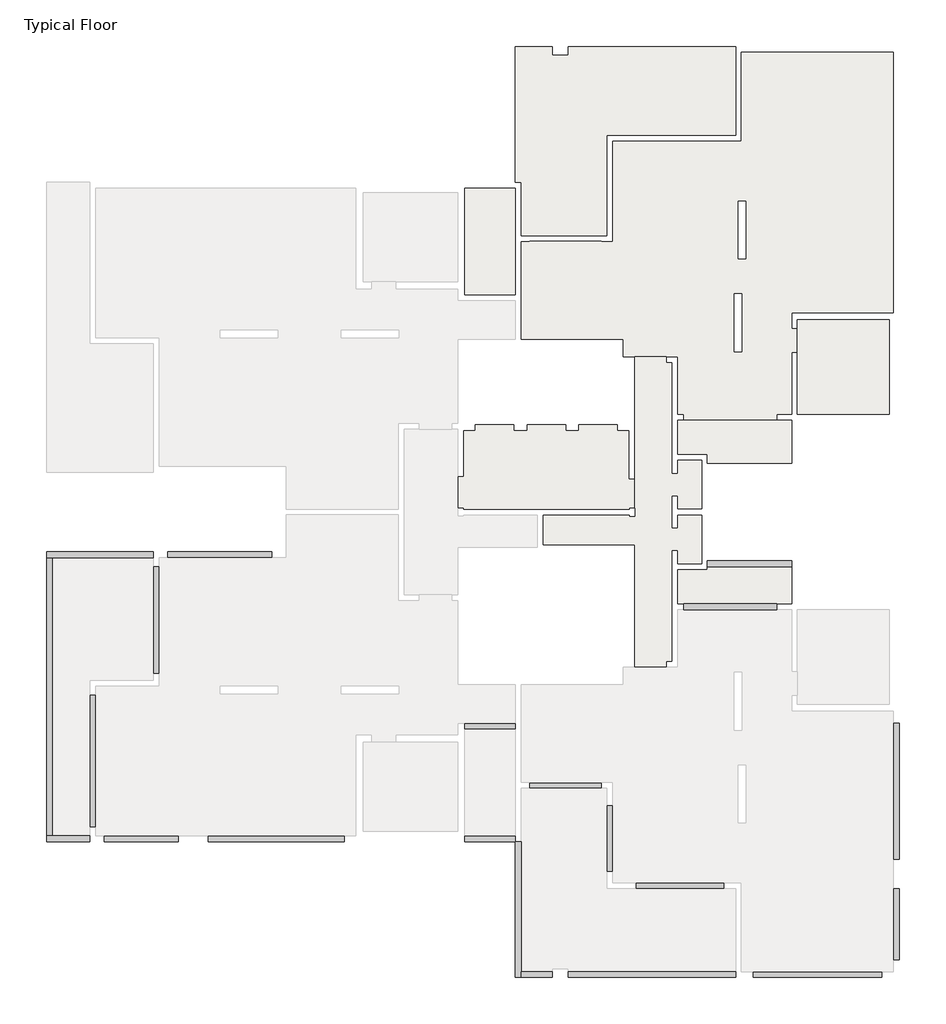
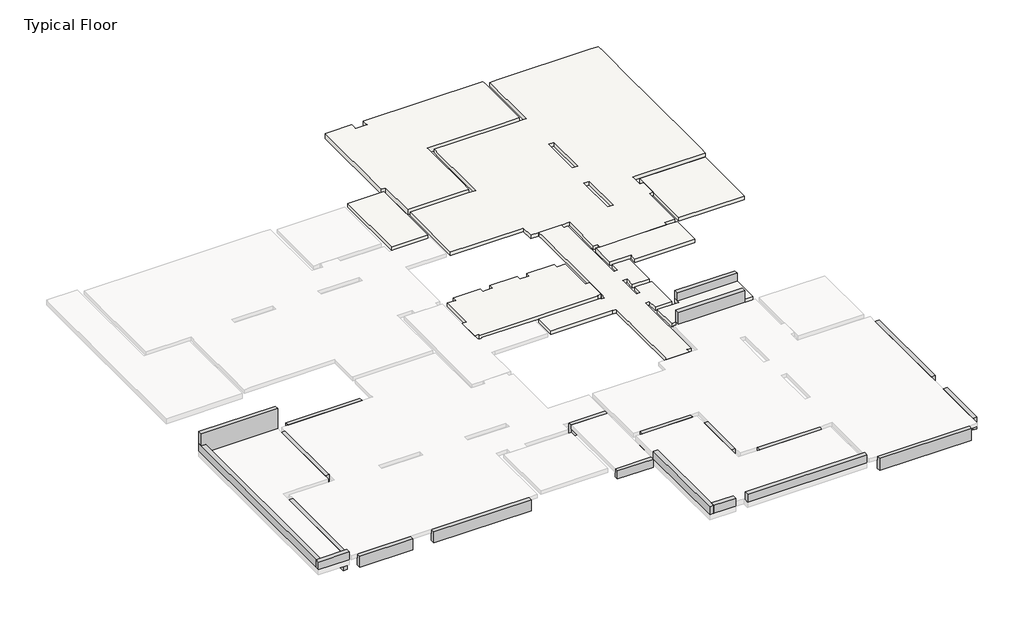
# One storey, part 2 of 2: 21 beams, 8 slabs.
"""IFC4 building model written with IfcOpenShell, lengths in millimetres."""

from ifc_helpers import new_model, si_unit, frame, origin, place, context, project, spatial, polyline, outline, extrude, faceted_brep, element, save

model = new_model("IFC4")

# Units and contexts
model_context = context("Model", 3, world=origin())
ifc_project = project(units=[si_unit("LENGTHUNIT", "METRE", prefix="MILLI")], contexts=[model_context])

# Site, building, storey
site = spatial("IfcSite", under=ifc_project)
building = spatial("IfcBuilding", under=site)
storey = spatial("IfcBuildingStorey", under=building, Name="Typical Floor", Elevation=3000.0)

# Beams
placement = place(None, origin())
element("IfcBeam", 1, ObjectType="Concrete Rectengular Beam : 20/40", at=placement, inside=storey, context=model_context, shape_type="Brep", body=[
    faceted_brep([(2246.4257984, -7661.3958819, 3000.0), (2246.4257984, -7661.3958819, 3400.0), (2446.4257984, -7661.3958819, 3400.0), (2446.4257984, -7661.3958819, 3000.0), (2246.4257984, -12260.9784014, 3400.0), (2446.4257984, -12260.9784014, 3400.0), (2446.4257984, -12060.9784014, 3400.0), (2446.4257984, -12260.9784014, 3000.0), (2446.4257984, -12060.9784014, 3000.0), (2246.4257984, -12260.9784014, 3000.0)], [[[0, 1, 2, 3]], [[2, 1, 4, 5, 6]], [[3, 2, 6, 5, 7, 8]], [[0, 3, 8, 7, 9]], [[1, 0, 9, 4]], [[5, 4, 9, 7]]]),
])
element("IfcBeam", 2, ObjectType="Concrete Rectengular Beam : 20/40", at=placement, inside=storey, context=model_context, shape_type="SweptSolid", body=[
    extrude(outline(polyline([(3495.6958179, -12060.9784014), (3495.6958179, -12260.9784014), (2446.4257984, -12260.9784014), (2446.4257984, -12060.9784014), (3495.6958179, -12060.9784014)])), frame((0.0, 0.0, 3000.0), z_axis=(0.0, 0.0, 1.0), x_axis=(1.0, 0.0, 0.0)), (0.0, 0.0, 1.0), 400.0),
])
element("IfcBeam", 3, ObjectType="Concrete Rectengular Beam : 20/40", at=placement, inside=storey, context=model_context, shape_type="SweptSolid", body=[
    extrude(outline(polyline([(9702.4292163, -12261.3104327), (4045.6958179, -12261.3104327), (4045.6958179, -12061.3104327), (9702.4292163, -12061.3104327), (9702.4292163, -12261.3104327)])), frame((0.0, 0.0, 3000.0), z_axis=(0.0, 0.0, 1.0), x_axis=(1.0, 0.0, 0.0)), (0.0, 0.0, 1.0), 400.0),
])
element("IfcBeam", 4, ObjectType="Concrete Rectengular Beam : 20/40", at=placement, inside=storey, context=model_context, shape_type="Brep", body=[
    faceted_brep([(2246.4257984, -7661.3958819, 3000.0), (2246.4257984, -7461.3958819, 3000.0), (542.9516773, -7461.3958819, 3000.0), (542.9516773, -7661.3958819, 3000.0), (542.9516773, -7661.3958819, 2600.0), (2246.4257984, -7661.3958819, 2600.0), (2246.4257984, -7461.3958819, 2600.0), (542.9516773, -7461.3958819, 2600.0), (2246.4257984, -7461.3958819, 2820.0), (542.9516773, -7461.3958819, 2820.0)], [[[0, 1, 2, 3]], [[3, 4, 5, 0]], [[6, 5, 4, 7]], [[1, 8, 6, 7, 9, 2]], [[1, 0, 5, 6, 8]], [[3, 2, 9, 7, 4]]]),
])
element("IfcBeam", 5, ObjectType="Concrete Rectengular Beam : 20/40", at=placement, inside=storey, context=model_context, shape_type="Brep", body=[
    faceted_brep([(-12154.2455884, -7461.3958819, 3000.0), (-12154.2455884, -7461.3958819, 3400.0), (-12154.2455884, -7661.3958819, 3400.0), (-12154.2455884, -7661.3958819, 3000.0), (-13414.2455884, -7461.3958819, 3400.0), (-13614.2455884, -7461.3958819, 3400.0), (-13614.2455884, -7661.3958819, 3400.0), (-13614.2455884, -7661.3958819, 3000.0), (-13614.2455884, -7461.3958819, 3000.0), (-13414.2455884, -7461.3958819, 3000.0)], [[[0, 1, 2, 3]], [[2, 1, 4, 5, 6]], [[3, 2, 6, 7]], [[0, 3, 7, 8, 9]], [[1, 0, 9, 8, 5, 4]], [[6, 5, 8, 7]]]),
])
element("IfcBeam", 6, ObjectType="Concrete Rectengular Beam : 20/40", at=placement, inside=storey, context=model_context, shape_type="Brep", body=[
    faceted_brep([(-13414.2455884, 2140.1763837, 3400.0), (-13614.2455884, 2140.1763837, 3400.0), (-13614.2455884, 1940.1763837, 3400.0), (-13614.2455884, -7461.3958819, 3400.0), (-13414.2455884, -7461.3958819, 3400.0), (-13414.2455884, 1940.1763837, 3400.0), (-13614.2455884, 2140.1763837, 3000.0), (-13614.2455884, -7461.3958819, 3000.0), (-13414.2455884, 2140.1763837, 3000.0), (-13414.2455884, 1940.1763837, 3000.0), (-13414.2455884, -7461.3958819, 3000.0)], [[[0, 1, 2, 3, 4, 5]], [[1, 6, 7, 3, 2]], [[6, 8, 9, 10, 7]], [[8, 0, 5, 4, 10, 9]], [[4, 3, 7, 10]], [[1, 0, 8, 6]]]),
])
element("IfcBeam", 7, ObjectType="Concrete Rectengular Beam : 20/40", at=placement, inside=storey, context=model_context, shape_type="SweptSolid", body=[
    extrude(outline(polyline([(8750.5859546, 1845.1910322), (11596.5527515, 1845.1910322), (11596.5527515, 1645.1910322), (8750.5859546, 1645.1910322), (8750.5859546, 1845.1910322)])), frame((0.0, 0.0, 3000.0), z_axis=(0.0, 0.0, 1.0), x_axis=(1.0, 0.0, 0.0)), (0.0, 0.0, 1.0), 400.0),
])
element("IfcBeam", 8, ObjectType="Concrete Rectengular Beam : 20/55", at=placement, inside=storey, context=model_context, shape_type="SweptSolid", body=[
    extrude(outline(polyline([(-7661.3958819, 2450.0), (-7661.3958819, 3000.0), (-7466.3958819, 3000.0), (-7466.3958819, 2820.0), (-7461.3958819, 2820.0), (-7461.3958819, 2450.0), (-7661.3958819, 2450.0)])), frame((-11654.2455884, 0.0, 0.0), z_axis=(1.0, 0.0, 0.0), x_axis=(0.0, 1.0, 0.0)), (0.0, 0.0, 1.0), 2499.5068359),
])
element("IfcBeam", 9, ObjectType="Concrete Rectengular Beam : 20/55", at=placement, inside=storey, context=model_context, shape_type="SweptSolid", body=[
    extrude(outline(polyline([(-7461.3958819, 2450.0), (-7661.3958819, 2450.0), (-7661.3958819, 3000.0), (-7466.3958819, 3000.0), (-7466.3958819, 2820.0), (-7461.3958819, 2820.0), (-7461.3958819, 2450.0)])), frame((-8149.7387524, 0.0, 0.0), z_axis=(1.0, 0.0, 0.0), x_axis=(0.0, 1.0, 0.0)), (0.0, 0.0, 1.0), 4602.6904297),
])
element("IfcBeam", 10, ObjectType="Concrete Rectengular Beam : 20/60", at=placement, inside=storey, context=model_context, shape_type="SweptSolid", body=[
    extrude(outline(polyline([(15247.1826343, -11661.3104327), (15047.1826343, -11661.3104327), (15047.1826343, -9252.3065264), (15247.1826343, -9252.3065264), (15247.1826343, -11661.3104327)])), frame((0.0, 0.0, 2400.0), z_axis=(0.0, 0.0, 1.0), x_axis=(1.0, 0.0, 0.0)), (0.0, 0.0, 1.0), 600.0),
])
element("IfcBeam", 11, ObjectType="Concrete Rectengular Beam : 20/60", at=placement, inside=storey, context=model_context, shape_type="SweptSolid", body=[
    extrude(outline(polyline([(15247.1826343, -8260.429085), (15047.1826343, -8260.429085), (15047.1826343, -3654.8187334), (15247.1826343, -3654.8187334), (15247.1826343, -8260.429085)])), frame((0.0, 0.0, 2400.0), z_axis=(0.0, 0.0, 1.0), x_axis=(1.0, 0.0, 0.0)), (0.0, 0.0, 1.0), 600.0),
])
element("IfcBeam", 12, ObjectType="Concrete Rectengular Beam : 20/60", at=placement, inside=storey, context=model_context, shape_type="Brep", body=[
    faceted_brep([(2246.4257984, -3861.3299639, 3000.0), (2246.4257984, -3661.3299639, 3000.0), (542.9516773, -3661.3299639, 3000.0), (542.9516773, -3861.3299639, 3000.0), (2246.4257984, -3861.3299639, 2400.0), (2246.4257984, -3861.3299639, 2820.0), (542.9516773, -3861.3299639, 2820.0), (542.9516773, -3861.3299639, 2400.0), (2246.4257984, -3661.3299639, 2400.0), (542.9516773, -3661.3299639, 2400.0), (2246.4257984, -3661.3299639, 2820.0)], [[[0, 1, 2, 3]], [[4, 5, 0, 3, 6, 7]], [[8, 4, 7, 9]], [[1, 10, 8, 9, 2]], [[1, 0, 5, 4, 8, 10]], [[3, 2, 9, 7, 6]]]),
])
element("IfcBeam", 13, ObjectType="Concrete Rectengular Beam : 20/60", at=placement, inside=storey, context=model_context, shape_type="SweptSolid", body=[
    extrude(outline(polyline([(11103.869646, 188.6553877), (7955.5859546, 188.6553877), (7955.5859546, 388.6553877), (11103.869646, 388.6553877), (11103.869646, 188.6553877)])), frame((0.0, 0.0, 3000.0), z_axis=(0.0, 0.0, 1.0), x_axis=(1.0, 0.0, 0.0)), (0.0, 0.0, 1.0), 600.0),
])
element("IfcBeam", 14, ObjectType="Concrete Rectengular Beam : 20/60", at=placement, inside=storey, context=model_context, shape_type="SweptSolid", body=[
    extrude(outline(polyline([(-12061.3104327, 2400.0), (-12261.3104327, 2400.0), (-12261.3104327, 3000.0), (-12066.3104327, 3000.0), (-12066.3104327, 2820.0), (-12061.3104327, 2820.0), (-12061.3104327, 2400.0)])), frame((10302.4292163, 0.0, 0.0), z_axis=(1.0, 0.0, 0.0), x_axis=(0.0, 1.0, 0.0)), (0.0, 0.0, 1.0), 4350.0610352),
])
element("IfcBeam", 15, ObjectType="Concrete Rectengular Beam : 20/85", at=placement, inside=storey, context=model_context, shape_type="Brep", body=[
    faceted_brep([(-12154.2455884, -7161.3958819, 3000.0), (-11954.2455884, -7161.3958819, 3000.0), (-11954.2455884, -2706.3494952, 3000.0), (-12154.2455884, -2706.3494952, 3000.0), (-11954.2455884, -7161.3958819, 2150.0), (-11954.2455884, -2706.3494952, 2150.0), (-12154.2455884, -7161.3958819, 2150.0), (-12154.2455884, -2706.3494952, 2150.0), (-12154.2455884, -2706.3494952, 2750.0), (-12154.2455884, -7161.3958819, 2750.0)], [[[0, 1, 2, 3]], [[1, 4, 5, 2]], [[4, 6, 7, 5]], [[0, 3, 8, 7, 6, 9]], [[1, 0, 9, 6, 4]], [[3, 2, 5, 7, 8]]]),
])
element("IfcBeam", 16, ObjectType="Concrete Rectengular Beam : 20/85", at=placement, inside=storey, context=model_context, shape_type="SweptSolid", body=[
    extrude(outline(polyline([(-5660.2777178, 2150.0), (-5860.2777178, 2150.0), (-5860.2777178, 3000.0), (-5665.2777178, 3000.0), (-5665.2777178, 2820.0), (-5660.2777178, 2820.0), (-5660.2777178, 2150.0)])), frame((2745.6201343, 0.0, 0.0), z_axis=(1.0, 0.0, 0.0), x_axis=(0.0, 1.0, 0.0)), (0.0, 0.0, 1.0), 2406.9848633),
])
element("IfcBeam", 17, ObjectType="Concrete Rectengular Beam : 20/85", at=placement, inside=storey, context=model_context, shape_type="Brep", body=[
    faceted_brep([(5545.4492359, -6456.8182452, 3000.0), (5345.4492359, -6456.8182452, 3000.0), (5345.4492359, -8661.9549639, 3000.0), (5545.4492359, -8661.9549639, 3000.0), (5545.4492359, -6456.8182452, 2150.0), (5545.4492359, -6456.8182452, 2820.0), (5545.4492359, -8661.9549639, 2820.0), (5545.4492359, -8661.9549639, 2150.0), (5345.4492359, -6456.8182452, 2150.0), (5345.4492359, -8661.9549639, 2150.0), (5345.4492359, -6456.8182452, 2750.0), (5345.4492359, -8661.9549639, 2750.0)], [[[0, 1, 2, 3]], [[4, 5, 0, 3, 6, 7]], [[8, 4, 7, 9]], [[2, 1, 10, 8, 9, 11]], [[1, 0, 5, 4, 8, 10]], [[3, 2, 11, 9, 7, 6]]]),
])
element("IfcBeam", 18, ObjectType="Concrete Rectengular Beam : 20/85", at=placement, inside=storey, context=model_context, shape_type="Brep", body=[
    faceted_brep([(6350.1123218, -9061.9549639, 3000.0), (6350.1123218, -9261.9549639, 3000.0), (9302.4292163, -9261.9549639, 3000.0), (9302.4292163, -9061.9549639, 3000.0), (9302.4292163, -9061.9549639, 2820.0), (9302.4292163, -9061.9549639, 2150.0), (6350.1123218, -9061.9549639, 2150.0), (6350.1123218, -9061.9549639, 2820.0), (6350.1123218, -9261.9549639, 2150.0), (9302.4292163, -9261.9549639, 2150.0), (6350.1123218, -9261.9549639, 2750.0), (9302.4292163, -9261.9549639, 2750.0)], [[[0, 1, 2, 3]], [[0, 3, 4, 5, 6, 7]], [[8, 6, 5, 9]], [[2, 1, 10, 8, 9, 11]], [[1, 0, 7, 6, 8, 10]], [[3, 2, 11, 9, 5, 4]]]),
])
element("IfcBeam", 19, ObjectType="Concrete Rectengular Beam : 20/85", at=placement, inside=storey, context=model_context, shape_type="Brep", body=[
    faceted_brep([(-9805.5395337, 1640.1763837, 3000.0), (-10005.5395337, 1640.1763837, 3000.0), (-10005.5395337, -1959.7284014, 3000.0), (-9805.5395337, -1959.7284014, 3000.0), (-10005.5395337, 1640.1763837, 2150.0), (-10005.5395337, -1959.7284014, 2150.0), (-9805.5395337, 1640.1763837, 2150.0), (-9805.5395337, -1959.7284014, 2150.0), (-9805.5395337, -1959.7284014, 2820.0), (-9805.5395337, 1640.1763837, 2820.0)], [[[0, 1, 2, 3]], [[1, 4, 5, 2]], [[4, 6, 7, 5]], [[0, 3, 8, 7, 6, 9]], [[1, 0, 9, 6, 4]], [[3, 2, 5, 7, 8]]]),
])
element("IfcBeam", 20, ObjectType="Concrete Rectengular Beam : 25/100", at=placement, inside=storey, context=model_context, shape_type="SweptSolid", body=[
    extrude(outline(polyline([(3000.0, -10005.5395337), (4000.0, -10005.5395337), (4000.0, -13614.2455884), (3400.0, -13614.2455884), (3400.0, -13414.2455884), (3000.0, -13414.2455884), (3000.0, -10005.5395337)])), frame((0.0, 1940.1763837, 0.0), z_axis=(0.0, 1.0, 0.0), x_axis=(0.0, 0.0, 1.0)), (0.0, 0.0, 1.0), 200.0),
])
element("IfcBeam", 21, ObjectType="Concrete Rectengular Beam : 25/100", at=placement, inside=storey, context=model_context, shape_type="Brep", body=[
    faceted_brep([(-9505.5395337, 2140.1763837, 3000.0), (-9505.5395337, 1940.1763837, 3000.0), (-5999.4457837, 1940.1763837, 3000.0), (-5999.4457837, 2140.1763837, 3000.0), (-9505.5395337, 2140.1763837, 2000.0), (-5999.4457837, 2140.1763837, 2000.0), (-9505.5395337, 1940.1763837, 2000.0), (-5999.4457837, 1940.1763837, 2000.0), (-9505.5395337, 1940.1763837, 2820.0), (-5999.4457837, 1940.1763837, 2820.0)], [[[0, 1, 2, 3]], [[4, 0, 3, 5]], [[6, 4, 5, 7]], [[2, 1, 8, 6, 7, 9]], [[1, 0, 4, 6, 8]], [[3, 2, 9, 7, 5]]]),
])

# Slabs
element("IfcSlab", 22, ObjectType="18", at=placement, inside=storey, context=model_context, shape_type="SweptSolid", body=[
    extrude(outline(polyline([(2246.4257984, 14441.4166181), (2246.4257984, 10841.3507002), (542.9516773, 10841.3507002), (542.9516773, 14441.4166181), (2246.4257984, 14441.4166181)])), frame((0.0, 0.0, 2820.0), z_axis=(0.0, 0.0, 1.0), x_axis=(1.0, 0.0, 0.0)), (0.0, 0.0, 1.0), 180.0),
])
element("IfcSlab", 23, ObjectType="18", at=placement, inside=storey, context=model_context, shape_type="Brep", body=[
    faceted_brep([(11596.5527515, 9690.0665205, 2820.0), (11796.5527515, 9690.0665205, 2820.0), (11796.5527515, 8889.8297041, 2820.0), (11596.5527515, 8889.8297041, 2820.0), (11596.5527515, 6791.3653486, 2820.0), (11103.869646, 6791.3653486, 2820.0), (11103.869646, 6591.3653486, 2820.0), (7955.5859546, 6591.3653486, 2820.0), (7955.5859546, 6791.3653486, 2820.0), (7751.2304859, 6791.3653486, 2820.0), (7751.2304859, 8540.3936689, 2820.0), (7751.2304859, 8740.3936689, 2820.0), (7351.2304859, 8740.3936689, 2820.0), (7351.2304859, 8739.7491377, 2820.0), (6296.4111499, 8739.7491377, 2820.0), (6296.4111499, 8740.0714033, 2820.0), (5901.4257984, 8740.0714033, 2820.0), (5901.4257984, 9337.0757978, 2820.0), (2446.4257984, 9337.0757978, 2820.0), (2446.4257984, 12640.2984541, 2820.0), (2745.6201343, 12640.2984541, 2820.0), (2745.6201343, 12645.2984541, 2820.0), (5152.6049976, 12645.2984541, 2820.0), (5152.6049976, 12640.2984541, 2820.0), (5545.4492359, 12640.2984541, 2820.0), (5545.4492359, 12840.2984541, 2820.0), (5545.4492359, 13436.8389814, 2820.0), (5545.4492359, 15641.9757002, 2820.0), (5545.4492359, 16041.9561689, 2820.0), (6350.1123218, 16041.9561689, 2820.0), (9302.4292163, 16041.9561689, 2820.0), (9902.4292163, 16041.9561689, 2820.0), (9902.4292163, 16241.9561689, 2820.0), (9902.4292163, 19041.3311689, 2820.0), (10302.4292163, 19041.3311689, 2820.0), (10302.4292163, 19046.3311689, 2820.0), (14652.4902515, 19046.3311689, 2820.0), (14652.4902515, 19041.3311689, 2820.0), (15047.1826343, 19041.3311689, 2820.0), (15047.1826343, 10239.8248212, 2820.0), (11596.5527515, 10239.8248212, 2820.0), (9796.8798999, 14005.4864423, 2820.0), (9796.8798999, 12062.9693525, 2820.0), (10046.8798999, 12062.9693525, 2820.0), (10046.8798999, 14005.4864423, 2820.0), (9656.2060718, 10871.4141767, 2820.0), (9656.2060718, 8920.2154462, 2820.0), (9906.2060718, 8920.2154462, 2820.0), (9906.2060718, 10871.4141767, 2820.0), (11796.5527515, 9690.0665205, 3000.0), (11596.5527515, 9690.0665205, 3000.0), (11596.5527515, 9690.7110517, 3000.0), (11596.5527515, 10239.8248212, 3000.0), (11796.5527515, 10239.8248212, 3000.0), (15047.1826343, 10239.8248212, 3000.0), (15047.1826343, 10634.8394697, 3000.0), (15047.1826343, 15240.4498212, 3000.0), (15047.1826343, 16232.3272627, 3000.0), (15047.1826343, 18641.3311689, 3000.0), (15047.1826343, 19041.3311689, 3000.0), (14652.4902515, 19041.3311689, 3000.0), (14652.4902515, 19046.3311689, 3000.0), (10302.4292163, 19046.3311689, 3000.0), (10302.4292163, 19041.3311689, 3000.0), (9902.4292163, 19041.3311689, 3000.0), (9902.4292163, 16241.9561689, 3000.0), (9902.4292163, 16041.9561689, 3000.0), (9302.4292163, 16041.9561689, 3000.0), (6350.1123218, 16041.9561689, 3000.0), (5545.4492359, 16041.9561689, 3000.0), (5545.4492359, 15641.9757002, 3000.0), (5545.4492359, 13436.8389814, 3000.0), (5545.4492359, 12840.2984541, 3000.0), (5545.4492359, 12640.2984541, 3000.0), (5152.6049976, 12640.2984541, 3000.0), (5152.6049976, 12645.2984541, 3000.0), (2745.6201343, 12645.2984541, 3000.0), (2745.6201343, 12640.2984541, 3000.0), (2446.4257984, 12640.2984541, 3000.0), (2446.4257984, 9337.0757978, 3000.0), (5701.4257984, 9337.0757978, 3000.0), (5901.4257984, 9337.0757978, 3000.0), (5901.4257984, 8740.0714033, 3000.0), (6296.4111499, 8740.0714033, 3000.0), (6296.4111499, 8739.7491377, 3000.0), (7351.2304859, 8739.7491377, 3000.0), (7351.2304859, 8740.3936689, 3000.0), (7751.2304859, 8740.3936689, 3000.0), (7751.2304859, 8540.3936689, 3000.0), (7751.2304859, 6791.3653486, 3000.0), (7955.5859546, 6791.3653486, 3000.0), (7955.5859546, 6591.3653486, 3000.0), (11103.869646, 6591.3653486, 3000.0), (11103.869646, 6791.3653486, 3000.0), (11596.5527515, 6791.3653486, 3000.0), (11596.5527515, 8889.8297041, 3000.0), (11796.5527515, 8889.8297041, 3000.0), (9796.8798999, 12062.9693525, 3000.0), (9796.8798999, 14005.4864423, 3000.0), (10046.8798999, 14005.4864423, 3000.0), (10046.8798999, 12062.9693525, 3000.0), (9656.2060718, 8920.2154462, 3000.0), (9656.2060718, 10871.4141767, 3000.0), (9906.2060718, 10871.4141767, 3000.0), (9906.2060718, 8920.2154462, 3000.0)], [[[0, 1, 2, 3, 4, 5, 6, 7, 8, 9, 10, 11, 12, 13, 14, 15, 16, 17, 18, 19, 20, 21, 22, 23, 24, 25, 26, 27, 28, 29, 30, 31, 32, 33, 34, 35, 36, 37, 38, 39, 40], [41, 42, 43, 44], [45, 46, 47, 48]], [[49, 50, 51, 52, 53, 54, 55, 56, 57, 58, 59, 60, 61, 62, 63, 64, 65, 66, 67, 68, 69, 70, 71, 72, 73, 74, 75, 76, 77, 78, 79, 80, 81, 82, 83, 84, 85, 86, 87, 88, 89, 90, 91, 92, 93, 94, 95, 96], [97, 98, 99, 100], [101, 102, 103, 104]], [[21, 76, 75, 22]], [[69, 28, 27, 26, 25, 24, 73, 72, 71, 70]], [[28, 69, 68, 67, 66, 31, 30, 29]], [[31, 66, 65, 64, 33, 32]], [[35, 62, 61, 36]], [[54, 39, 38, 59, 58, 57, 56, 55]], [[50, 0, 40, 52, 51]], [[1, 0, 50, 49]], [[1, 49, 96, 2]], [[3, 95, 94, 4]], [[87, 11, 10, 9, 89, 88]], [[84, 14, 13, 85]], [[16, 82, 81, 17]], [[18, 79, 78, 19]], [[77, 20, 19, 78]], [[20, 77, 76, 21]], [[73, 24, 23, 74]], [[74, 23, 22, 75]], [[41, 98, 97, 42]], [[43, 100, 99, 44]], [[42, 97, 100, 43]], [[98, 41, 44, 99]], [[45, 102, 101, 46]], [[47, 104, 103, 48]], [[46, 101, 104, 47]], [[102, 45, 48, 103]], [[39, 54, 53, 52, 40]], [[95, 3, 2, 96]], [[15, 83, 82, 16]], [[83, 15, 14, 84]], [[11, 87, 86, 12]], [[12, 86, 85, 13]], [[8, 90, 89, 9]], [[5, 4, 94, 93]], [[6, 5, 93, 92]], [[7, 6, 92, 91]], [[90, 8, 7, 91]], [[17, 81, 80, 79, 18]], [[63, 34, 33, 64]], [[34, 63, 62, 35]], [[37, 60, 59, 38]], [[60, 37, 36, 61]]]),
])
element("IfcSlab", 24, ObjectType="18", at=placement, inside=storey, context=model_context, shape_type="Brep", body=[
    faceted_brep([(11596.5527515, 6591.3653486, 2820.0), (11596.5527515, 5134.8297041, 2820.0), (8750.5859546, 5134.8297041, 2820.0), (8750.5859546, 5241.3702314, 2820.0), (8750.5859546, 5441.3702314, 2820.0), (7751.2304859, 5441.3702314, 2820.0), (7751.2304859, 6591.3653486, 2820.0), (7955.5859546, 6591.3653486, 2820.0), (11103.869646, 6591.3653486, 2820.0), (11596.5527515, 5134.8297041, 3000.0), (11596.5527515, 5334.8297041, 3000.0), (11596.5527515, 6591.3653486, 3000.0), (11103.869646, 6591.3653486, 3000.0), (7955.5859546, 6591.3653486, 3000.0), (7751.2304859, 6591.3653486, 3000.0), (7751.2304859, 5441.3702314, 3000.0), (8750.5859546, 5441.3702314, 3000.0), (8750.5859546, 5334.8297041, 3000.0), (8750.5859546, 5241.3702314, 3000.0), (8750.5859546, 5134.8297041, 3000.0)], [[[0, 1, 2, 3, 4, 5, 6, 7, 8]], [[9, 10, 11, 12, 13, 14, 15, 16, 17, 18, 19]], [[1, 0, 11, 10, 9]], [[2, 1, 9, 19]], [[2, 19, 18, 17, 16, 4, 3]], [[5, 4, 16, 15]], [[6, 5, 15, 14]], [[0, 8, 7, 6, 14, 13, 12, 11]]]),
])
element("IfcSlab", 25, ObjectType="18", at=placement, inside=storey, context=model_context, shape_type="Brep", body=[
    faceted_brep([(11596.5527515, 1845.1910322, 2820.0), (11596.5527515, 388.6553877, 2820.0), (11103.869646, 388.6553877, 2820.0), (7955.5859546, 388.6553877, 2820.0), (7751.2304859, 388.6553877, 2820.0), (7751.2304859, 1538.6505048, 2820.0), (8750.5859546, 1538.6505048, 2820.0), (8750.5859546, 1738.6505048, 2820.0), (8750.5859546, 1845.1910322, 2820.0), (11596.5527515, 388.6553877, 3000.0), (11596.5527515, 1645.1910322, 3000.0), (11596.5527515, 1845.1910322, 3000.0), (8750.5859546, 1845.1910322, 3000.0), (8750.5859546, 1738.6505048, 3000.0), (8750.5859546, 1645.1910322, 3000.0), (8750.5859546, 1538.6505048, 3000.0), (7751.2304859, 1538.6505048, 3000.0), (7751.2304859, 388.6553877, 3000.0), (7955.5859546, 388.6553877, 3000.0), (11103.869646, 388.6553877, 3000.0)], [[[0, 1, 2, 3, 4, 5, 6, 7, 8]], [[9, 10, 11, 12, 13, 14, 15, 16, 17, 18, 19]], [[1, 0, 11, 10, 9]], [[0, 8, 12, 11]], [[6, 15, 14, 13, 12, 8, 7]], [[6, 5, 16, 15]], [[5, 4, 17, 16]], [[4, 3, 2, 1, 9, 19, 18, 17]]]),
])
element("IfcSlab", 26, ObjectType="18", at=placement, inside=storey, context=model_context, shape_type="Brep", body=[
    faceted_brep([(14897.1826343, 9989.8248212, 2820.0), (14897.1826343, 6791.445915, 2820.0), (11796.5527515, 6791.445915, 2820.0), (11796.5527515, 8889.1851728, 2820.0), (11796.5527515, 8889.8297041, 2820.0), (11796.5527515, 9690.0665205, 2820.0), (11796.5527515, 9989.8248212, 2820.0), (14897.1826343, 6791.445915, 3000.0), (14897.1826343, 9989.8248212, 3000.0), (11796.5527515, 9989.8248212, 3000.0), (11796.5527515, 9690.7110517, 3000.0), (11796.5527515, 9690.0665205, 3000.0), (11796.5527515, 8889.8297041, 3000.0), (11796.5527515, 8889.1851728, 3000.0), (11796.5527515, 6791.445915, 3000.0)], [[[0, 1, 2, 3, 4, 5, 6]], [[7, 8, 9, 10, 11, 12, 13, 14]], [[1, 0, 8, 7]], [[2, 1, 7, 14]], [[2, 14, 13, 12, 11, 10, 9, 6, 5, 4, 3]], [[0, 6, 9, 8]]]),
])
element("IfcSlab", 27, ObjectType="18", at=placement, inside=storey, context=model_context, shape_type="Brep", body=[
    faceted_brep([(7351.2304859, -1560.3826983, 2820.0), (7351.2304859, -1759.7284014, 2820.0), (6296.4111499, -1759.7284014, 2820.0), (6296.4111499, -1559.7284014, 2820.0), (6296.4111499, 2389.7735517, 2820.0), (6096.4111499, 2389.7735517, 2820.0), (6096.4111499, 2389.4512861, 2820.0), (3197.0654468, 2389.4512861, 2820.0), (3197.0654468, 3385.0909345, 2820.0), (6101.7382984, 3385.0909345, 2820.0), (6101.7382984, 3335.0909345, 2820.0), (6301.7382984, 3335.0909345, 2820.0), (6301.7382984, 3635.0909345, 2820.0), (6296.4111499, 3635.0909345, 2820.0), (6296.4111499, 4590.2471845, 2820.0), (6296.4111499, 8390.0714033, 2820.0), (6296.4111499, 8739.7491377, 2820.0), (7351.2304859, 8739.7491377, 2820.0), (7351.2304859, 8540.3936689, 2820.0), (7551.2304859, 8540.3936689, 2820.0), (7551.2304859, 4780.3936689, 2820.0), (7751.2304859, 4780.3936689, 2820.0), (7751.2304859, 5241.3702314, 2820.0), (8550.5859546, 5241.3702314, 2820.0), (8550.5859546, 3593.6505048, 2820.0), (7750.5859546, 3593.6505048, 2820.0), (7750.5859546, 4036.3702314, 2820.0), (7550.5859546, 4036.3702314, 2820.0), (7550.5859546, 2943.6505048, 2820.0), (7750.5859546, 2943.6505048, 2820.0), (7750.5859546, 3386.3702314, 2820.0), (8550.5859546, 3386.3702314, 2820.0), (8550.5859546, 1738.6505048, 2820.0), (7751.2304859, 1738.6505048, 2820.0), (7751.2304859, 2199.6270673, 2820.0), (7551.2304859, 2199.6270673, 2820.0), (7551.2304859, -1560.3826983, 2820.0), (7351.2304859, -1759.7284014, 3000.0), (7351.2304859, -1560.3826983, 3000.0), (7551.2304859, -1560.3826983, 3000.0), (7551.2304859, 2199.6270673, 3000.0), (7751.2304859, 2199.6270673, 3000.0), (7751.2304859, 1738.6505048, 3000.0), (8550.5859546, 1738.6505048, 3000.0), (8550.5859546, 3386.3702314, 3000.0), (7750.5859546, 3386.3702314, 3000.0), (7750.5859546, 2943.6505048, 3000.0), (7550.5859546, 2943.6505048, 3000.0), (7550.5859546, 4036.3702314, 3000.0), (7750.5859546, 4036.3702314, 3000.0), (7750.5859546, 3593.6505048, 3000.0), (8550.5859546, 3593.6505048, 3000.0), (8550.5859546, 5241.3702314, 3000.0), (7751.2304859, 5241.3702314, 3000.0), (7751.2304859, 4780.3936689, 3000.0), (7551.2304859, 4780.3936689, 3000.0), (7551.2304859, 8540.3936689, 3000.0), (7351.2304859, 8540.3936689, 3000.0), (7351.2304859, 8739.7491377, 3000.0), (6296.4111499, 8739.7491377, 3000.0), (6296.4111499, 8390.0714033, 3000.0), (6296.4111499, 4590.2471845, 3000.0), (6296.4111499, 3635.0909345, 3000.0), (6301.7382984, 3635.0909345, 3000.0), (6301.7382984, 3335.0909345, 3000.0), (6101.7382984, 3335.0909345, 3000.0), (6101.7382984, 3385.0909345, 3000.0), (3197.0654468, 3385.0909345, 3000.0), (3197.0654468, 2389.4512861, 3000.0), (6096.4111499, 2389.4512861, 3000.0), (6096.4111499, 2389.7735517, 3000.0), (6296.4111499, 2389.7735517, 3000.0), (6296.4111499, -1559.7284014, 3000.0), (6296.4111499, -1759.7284014, 3000.0)], [[[0, 1, 2, 3, 4, 5, 6, 7, 8, 9, 10, 11, 12, 13, 14, 15, 16, 17, 18, 19, 20, 21, 22, 23, 24, 25, 26, 27, 28, 29, 30, 31, 32, 33, 34, 35, 36]], [[37, 38, 39, 40, 41, 42, 43, 44, 45, 46, 47, 48, 49, 50, 51, 52, 53, 54, 55, 56, 57, 58, 59, 60, 61, 62, 63, 64, 65, 66, 67, 68, 69, 70, 71, 72, 73]], [[1, 0, 38, 37]], [[2, 1, 37, 73]], [[2, 73, 72, 71, 4, 3]], [[68, 7, 6, 69]], [[8, 7, 68, 67]], [[9, 8, 67, 66]], [[10, 9, 66, 65]], [[11, 10, 65, 64]], [[12, 11, 64, 63]], [[13, 12, 63, 62]], [[14, 13, 62, 61]], [[14, 61, 60, 59, 16, 15]], [[17, 16, 59, 58]], [[18, 17, 58, 57]], [[19, 18, 57, 56]], [[20, 19, 56, 55]], [[21, 20, 55, 54]], [[22, 21, 54, 53]], [[23, 22, 53, 52]], [[24, 23, 52, 51]], [[25, 24, 51, 50]], [[26, 25, 50, 49]], [[27, 26, 49, 48]], [[28, 27, 48, 47]], [[29, 28, 47, 46]], [[30, 29, 46, 45]], [[31, 30, 45, 44]], [[32, 31, 44, 43]], [[33, 32, 43, 42]], [[34, 33, 42, 41]], [[35, 34, 41, 40]], [[36, 35, 40, 39]], [[0, 36, 39, 38]], [[5, 70, 69, 6]], [[70, 5, 4, 71]]]),
])
element("IfcSlab", 28, ObjectType="18", at=placement, inside=storey, context=model_context, shape_type="SweptSolid", body=[
    extrude(outline(polyline([(306.4257984, 4687.0757978), (506.4257984, 4687.0757978), (506.4257984, 6239.7589033), (900.756853, 6239.7589033), (900.756853, 6439.7589033), (2196.5063648, 6439.7589033), (2196.5063648, 6239.7589033), (2645.7812671, 6239.7589033), (2645.7812671, 6439.7589033), (3950.197771, 6439.7589033), (3950.197771, 6239.7589033), (4397.3022632, 6239.7589033), (4397.3022632, 6439.7589033), (5697.3779468, 6439.7589033), (5697.3779468, 6239.7589033), (6096.4111499, 6239.7589033), (6096.4111499, 4590.2471845), (6296.4111499, 4590.2471845), (6296.4111499, 3635.0909345), (6101.7382984, 3635.0909345), (6101.7382984, 3585.0909345), (501.7382984, 3585.0909345), (501.7382984, 3635.0909345), (306.4257984, 3635.0909345), (306.4257984, 4687.0757978)])), frame((0.0, 0.0, 2820.0), z_axis=(0.0, 0.0, 1.0), x_axis=(1.0, 0.0, 0.0)), (0.0, 0.0, 1.0), 180.0),
])
element("IfcSlab", 29, ObjectType="25", at=placement, inside=storey, context=model_context, shape_type="Brep", body=[
    faceted_brep([(2246.4257984, 19240.9991377, 2750.0), (3495.6958179, 19240.9991377, 2750.0), (3495.6958179, 18940.9991377, 2750.0), (4045.6958179, 18940.9991377, 2750.0), (4045.6958179, 19240.9991377, 2750.0), (4045.6958179, 19241.3311689, 2750.0), (9702.4292163, 19241.3311689, 2750.0), (9702.4292163, 16241.9561689, 2750.0), (9302.4292163, 16241.9561689, 2750.0), (6350.1123218, 16241.9561689, 2750.0), (5545.4492359, 16241.9561689, 2750.0), (5345.4492359, 16241.9561689, 2750.0), (5345.4492359, 15641.9757002, 2750.0), (5345.4492359, 13436.8389814, 2750.0), (5345.4492359, 12840.2984541, 2750.0), (2446.4257984, 12840.2984541, 2750.0), (2446.4257984, 14641.4166181, 2750.0), (2246.4257984, 14641.4166181, 2750.0), (3495.6958179, 19240.9991377, 3000.0), (2446.4257984, 19240.9991377, 3000.0), (2246.4257984, 19240.9991377, 3000.0), (2246.4257984, 14641.4166181, 3000.0), (2446.4257984, 14641.4166181, 3000.0), (2446.4257984, 12840.2984541, 3000.0), (2745.6201343, 12840.2984541, 3000.0), (5152.6049976, 12840.2984541, 3000.0), (5345.4492359, 12840.2984541, 3000.0), (5345.4492359, 13436.8389814, 3000.0), (5345.4492359, 15641.9757002, 3000.0), (5345.4492359, 16241.9561689, 3000.0), (5545.4492359, 16241.9561689, 3000.0), (6350.1123218, 16241.9561689, 3000.0), (9302.4292163, 16241.9561689, 3000.0), (9702.4292163, 16241.9561689, 3000.0), (9702.4292163, 19041.3311689, 3000.0), (9702.4292163, 19241.3311689, 3000.0), (4045.6958179, 19241.3311689, 3000.0), (4045.6958179, 19240.9991377, 3000.0), (4045.6958179, 19041.3311689, 3000.0), (4045.6958179, 18940.9991377, 3000.0), (3495.6958179, 18940.9991377, 3000.0), (3495.6958179, 19040.9991377, 3000.0)], [[[0, 1, 2, 3, 4, 5, 6, 7, 8, 9, 10, 11, 12, 13, 14, 15, 16, 17]], [[18, 19, 20, 21, 22, 23, 24, 25, 26, 27, 28, 29, 30, 31, 32, 33, 34, 35, 36, 37, 38, 39, 40, 41]], [[1, 0, 20, 19, 18]], [[2, 1, 18, 41, 40]], [[3, 2, 40, 39]], [[3, 39, 38, 37, 36, 5, 4]], [[6, 5, 36, 35]], [[7, 6, 35, 34, 33]], [[7, 33, 32, 31, 30, 29, 11, 10, 9, 8]], [[11, 29, 28, 27, 26, 14, 13, 12]], [[15, 14, 26, 25, 24, 23]], [[0, 17, 21, 20]], [[16, 15, 23, 22]], [[17, 16, 22, 21]]]),
])

save(model, "model.ifc")

# Revit data of these elements
# Type "Concrete Rectengular Beam : 20/40"
#   Keynote = "09000"
#   Length [instance default] = 152.4 cm
#   b = 20 cm
#   h = 40 cm
#   Structural Material [instance default] = Concrete
#   Assembly Code = ""
# Type "Concrete Rectengular Beam : 20/55"
#   Length [instance default] = 152.4 cm
#   b = 20 cm
#   h = 55 cm
#   Structural Material [instance default] = Concrete
#   Assembly Code = ""
# Type "Concrete Rectengular Beam : 20/60"
#   Length [instance default] = 152.4 cm
#   b = 20 cm
#   h = 60 cm
#   Structural Material [instance default] = Concrete
#   Assembly Code = ""
# Type "Concrete Rectengular Beam : 20/85"
#   Length [instance default] = 152.4 cm
#   b = 20 cm
#   h = 85 cm
#   Structural Material [instance default] = Concrete
#   Assembly Code = ""
# Type "Concrete Rectengular Beam : 25/100"
#   Length [instance default] = 152.4 cm
#   b = 20 cm
#   h = 100 cm
#   Structural Material [instance default] = Concrete
#   Assembly Code = ""
# Type "18"
#   Function = 0
#   Layers, outside or top first: 18 cm "Concrete" (function 1)
# Type "25"
#   Function = 0
#   Layers, outside or top first: 25 cm "Concrete" (function 1)
# Element 1 (IfcBeam, "Concrete Rectengular Beam : 20/40")
#   Comments = ""
#   Mark = "B8"
#   SOFiSTiK_AMG_Comments = ""
#   SOFiSTiK_AMG_Scheduled = yes
#   SOFiSTiK_AMG_Adjusted = yes
#   Structural Material = Concrete
#   Phase Created = New Construction
#   Materials on its faces: "Concrete"
# Element 2 (IfcBeam, "Concrete Rectengular Beam : 20/40")
#   Comments = ""
#   Mark = "B9"
#   SOFiSTiK_AMG_Comments = ""
#   SOFiSTiK_AMG_Scheduled = yes
#   SOFiSTiK_AMG_Adjusted = yes
#   Structural Material = Concrete
#   Phase Created = New Construction
#   Materials on its faces: "Concrete"
# Element 3 (IfcBeam, "Concrete Rectengular Beam : 20/40")
#   Comments = ""
#   Mark = "B10"
#   SOFiSTiK_AMG_Comments = ""
#   SOFiSTiK_AMG_Scheduled = yes
#   SOFiSTiK_AMG_Adjusted = yes
#   Structural Material = Concrete
#   Phase Created = New Construction
#   Materials on its faces: "Concrete"
# Element 4 (IfcBeam, "Concrete Rectengular Beam : 20/40")
#   Comments = ""
#   Mark = "B11"
#   SOFiSTiK_AMG_Comments = ""
#   SOFiSTiK_AMG_Scheduled = yes
#   SOFiSTiK_AMG_Adjusted = yes
#   Structural Material = Concrete
#   Phase Created = New Construction
#   Materials on its faces: "Concrete"
# Element 5 (IfcBeam, "Concrete Rectengular Beam : 20/40")
#   Comments = ""
#   Mark = "B12"
#   SOFiSTiK_AMG_Comments = ""
#   SOFiSTiK_AMG_Scheduled = yes
#   SOFiSTiK_AMG_Adjusted = yes
#   Structural Material = Concrete
#   Phase Created = New Construction
#   Materials on its faces: "Concrete"
# Element 6 (IfcBeam, "Concrete Rectengular Beam : 20/40")
#   Comments = ""
#   Mark = "B13"
#   SOFiSTiK_AMG_Comments = ""
#   SOFiSTiK_AMG_Scheduled = yes
#   SOFiSTiK_AMG_Adjusted = yes
#   Structural Material = Concrete
#   Phase Created = New Construction
#   Materials on its faces: "Concrete"
# Element 7 (IfcBeam, "Concrete Rectengular Beam : 20/40")
#   Comments = ""
#   Mark = "B14"
#   SOFiSTiK_AMG_Comments = ""
#   SOFiSTiK_AMG_Scheduled = yes
#   SOFiSTiK_AMG_Adjusted = yes
#   Structural Material = Concrete
#   Phase Created = New Construction
#   Materials on its faces: "Concrete"
# Element 8 (IfcBeam, "Concrete Rectengular Beam : 20/55")
#   Comments = ""
#   Mark = "B17"
#   SOFiSTiK_AMG_Comments = ""
#   SOFiSTiK_AMG_Scheduled = yes
#   SOFiSTiK_AMG_Adjusted = yes
#   Structural Material = Concrete
#   Phase Created = New Construction
#   Materials on its faces: "Concrete"
# Element 9 (IfcBeam, "Concrete Rectengular Beam : 20/55")
#   Comments = ""
#   Mark = "B18"
#   SOFiSTiK_AMG_Comments = ""
#   SOFiSTiK_AMG_Scheduled = yes
#   SOFiSTiK_AMG_Adjusted = yes
#   Structural Material = Concrete
#   Phase Created = New Construction
#   Materials on its faces: "Concrete"
# Element 10 (IfcBeam, "Concrete Rectengular Beam : 20/60")
#   Comments = ""
#   Mark = "B25"
#   SOFiSTiK_AMG_Comments = ""
#   SOFiSTiK_AMG_Scheduled = yes
#   SOFiSTiK_AMG_Adjusted = yes
#   Structural Material = Concrete
#   Phase Created = New Construction
#   Materials on its faces: "Concrete"
# Element 11 (IfcBeam, "Concrete Rectengular Beam : 20/60")
#   Comments = ""
#   Mark = "B26"
#   SOFiSTiK_AMG_Comments = ""
#   SOFiSTiK_AMG_Scheduled = yes
#   SOFiSTiK_AMG_Adjusted = yes
#   Structural Material = Concrete
#   Phase Created = New Construction
#   Materials on its faces: "Concrete"
# Element 12 (IfcBeam, "Concrete Rectengular Beam : 20/60")
#   Comments = ""
#   Mark = "B27"
#   SOFiSTiK_AMG_Comments = ""
#   SOFiSTiK_AMG_Scheduled = yes
#   SOFiSTiK_AMG_Adjusted = yes
#   Structural Material = Concrete
#   Phase Created = New Construction
#   Materials on its faces: "Concrete"
# Element 13 (IfcBeam, "Concrete Rectengular Beam : 20/60")
#   Comments = ""
#   Mark = "B28"
#   SOFiSTiK_AMG_Comments = ""
#   SOFiSTiK_AMG_Scheduled = yes
#   SOFiSTiK_AMG_Adjusted = yes
#   Structural Material = Concrete
#   Phase Created = New Construction
#   Materials on its faces: "Concrete"
# Element 14 (IfcBeam, "Concrete Rectengular Beam : 20/60")
#   Comments = ""
#   Mark = "B29"
#   SOFiSTiK_AMG_Comments = ""
#   SOFiSTiK_AMG_Scheduled = yes
#   SOFiSTiK_AMG_Adjusted = yes
#   Structural Material = Concrete
#   Phase Created = New Construction
#   Materials on its faces: "Concrete"
# Element 15 (IfcBeam, "Concrete Rectengular Beam : 20/85")
#   Comments = ""
#   Mark = "B35"
#   SOFiSTiK_AMG_Comments = ""
#   SOFiSTiK_AMG_Scheduled = yes
#   SOFiSTiK_AMG_Adjusted = yes
#   Structural Material = Concrete
#   Phase Created = New Construction
#   Materials on its faces: "Concrete"
# Element 16 (IfcBeam, "Concrete Rectengular Beam : 20/85")
#   Comments = ""
#   Mark = "B36"
#   SOFiSTiK_AMG_Comments = ""
#   SOFiSTiK_AMG_Scheduled = yes
#   SOFiSTiK_AMG_Adjusted = yes
#   Structural Material = Concrete
#   Phase Created = New Construction
#   Materials on its faces: "Concrete"
# Element 17 (IfcBeam, "Concrete Rectengular Beam : 20/85")
#   Comments = ""
#   Mark = "B37"
#   SOFiSTiK_AMG_Comments = ""
#   SOFiSTiK_AMG_Scheduled = yes
#   SOFiSTiK_AMG_Adjusted = yes
#   Structural Material = Concrete
#   Phase Created = New Construction
#   Materials on its faces: "Concrete"
# Element 18 (IfcBeam, "Concrete Rectengular Beam : 20/85")
#   Comments = ""
#   Mark = "B38"
#   SOFiSTiK_AMG_Comments = ""
#   SOFiSTiK_AMG_Scheduled = yes
#   SOFiSTiK_AMG_Adjusted = yes
#   Structural Material = Concrete
#   Phase Created = New Construction
#   Materials on its faces: "Concrete"
# Element 19 (IfcBeam, "Concrete Rectengular Beam : 20/85")
#   Comments = ""
#   Mark = "B39"
#   SOFiSTiK_AMG_Comments = ""
#   SOFiSTiK_AMG_Scheduled = yes
#   SOFiSTiK_AMG_Adjusted = yes
#   Structural Material = Concrete
#   Phase Created = New Construction
#   Materials on its faces: "Concrete"
# Element 20 (IfcBeam, "Concrete Rectengular Beam : 25/100")
#   Comments = ""
#   Mark = "B42"
#   SOFiSTiK_AMG_Comments = ""
#   SOFiSTiK_AMG_Scheduled = yes
#   SOFiSTiK_AMG_Adjusted = yes
#   Structural Material = Concrete
#   Phase Created = New Construction
#   Materials on its faces: "Concrete"
# Element 21 (IfcBeam, "Concrete Rectengular Beam : 25/100")
#   Comments = ""
#   Mark = "B43"
#   SOFiSTiK_AMG_Comments = ""
#   SOFiSTiK_AMG_Scheduled = yes
#   SOFiSTiK_AMG_Adjusted = yes
#   Structural Material = Concrete
#   Phase Created = New Construction
#   Materials on its faces: "Concrete"
# Element 22 (IfcSlab, "18")
#   Mark = "S7"
#   SOFiSTiK_AMG_Comments = ""
#   Height Offset From Level = 0 cm
#   built-in parameter 1001954 = 1
#   SOFiSTiK_AMG_Scheduled = yes
#   SOFiSTiK_AMG_Adjusted = yes
#   Phase Created = New Construction
#   Materials on its faces: "Concrete"
# Element 23 (IfcSlab, "18")
#   Mark = "S8"
#   SOFiSTiK_AMG_Comments = ""
#   built-in parameter 1001955 = 1.5708 (stored number, unit not read)
#   Height Offset From Level = 0 cm
#   built-in parameter 1001954 = 1
#   SOFiSTiK_AMG_Scheduled = yes
#   SOFiSTiK_AMG_Adjusted = yes
#   Phase Created = New Construction
#   Materials on its faces: "Concrete"
# Element 24 (IfcSlab, "18")
#   Mark = "S9"
#   SOFiSTiK_AMG_Comments = ""
#   Height Offset From Level = 0 cm
#   built-in parameter 1001954 = 1
#   SOFiSTiK_AMG_Scheduled = yes
#   SOFiSTiK_AMG_Adjusted = yes
#   Phase Created = New Construction
#   Materials on its faces: "Concrete"
# Element 25 (IfcSlab, "18")
#   Mark = "S15"
#   SOFiSTiK_AMG_Comments = ""
#   Height Offset From Level = 0 cm
#   built-in parameter 1001954 = 1
#   SOFiSTiK_AMG_Scheduled = yes
#   SOFiSTiK_AMG_Adjusted = yes
#   Phase Created = New Construction
#   Materials on its faces: "Concrete"
# Element 26 (IfcSlab, "18")
#   Mark = "S16"
#   SOFiSTiK_AMG_Comments = ""
#   Height Offset From Level = 0 cm
#   built-in parameter 1001954 = 1
#   SOFiSTiK_AMG_Scheduled = yes
#   SOFiSTiK_AMG_Adjusted = yes
#   Phase Created = New Construction
#   Materials on its faces: "Concrete"
# Element 27 (IfcSlab, "18")
#   Mark = "S17"
#   SOFiSTiK_AMG_Comments = ""
#   built-in parameter 1001955 = 1.5708 (stored number, unit not read)
#   Height Offset From Level = 0 cm
#   built-in parameter 1001954 = 1
#   SOFiSTiK_AMG_Scheduled = yes
#   SOFiSTiK_AMG_Adjusted = yes
#   Phase Created = New Construction
#   Materials on its faces: "Concrete"
# Element 28 (IfcSlab, "18")
#   Mark = "S19"
#   SOFiSTiK_AMG_Comments = ""
#   built-in parameter 1001955 = 1.5708 (stored number, unit not read)
#   Height Offset From Level = 0 cm
#   built-in parameter 1001954 = 1
#   SOFiSTiK_AMG_Scheduled = yes
#   SOFiSTiK_AMG_Adjusted = yes
#   Phase Created = New Construction
#   Materials on its faces: "Concrete"
# Element 29 (IfcSlab, "25")
#   Mark = "S2"
#   SOFiSTiK_AMG_Comments = ""
#   built-in parameter 1001955 = 1.5708 (stored number, unit not read)
#   Height Offset From Level = 0 cm
#   built-in parameter 1001954 = 1
#   SOFiSTiK_AMG_Scheduled = yes
#   SOFiSTiK_AMG_Adjusted = no
#   Phase Created = New Construction
#   Materials on its faces: "Concrete"
# Materials
#   "Concrete": class "Concrete", colour RGB 192 192 192, transparency 0, Keynote = "01000", Description = "Cast-in-place concrete", Cost = 0
